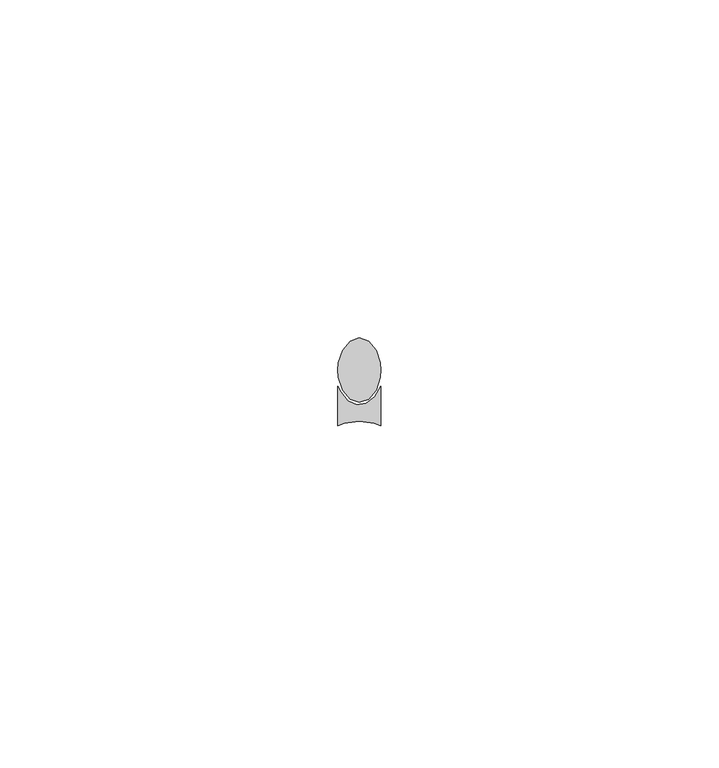
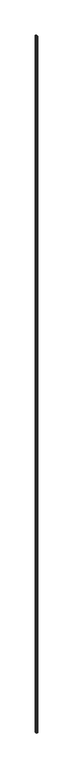
"""IFC4 building model written with IfcOpenShell, lengths in millimetres: proxy geometry, Generic Models 11:Generic Models 1:306267:Generic Models 1:306267 : Generic Models 11:Generic Models 1:306267:300405:Generic Models 1:306267:Generic Models 1:306267 : Generic Models 11:Generic Models 1:306267:300405 : Generic Models 11:Generic Models 1:306267:Generic Models 1:306267 : Generic Models 11:Generic Models 1:306267:300405:4 : Generic Models 11:Generic Models 1:306267:Generic Models 1:306267 : Generic Models 11:Generic Models 1:306267:300405:Generic Models 1:306267:Generic Models 1:306267 : Generic Models 11:Generic Models 1:306267:300405 : Generic Models 11:Generic Models 1:306267:Generic Models 1:306267 : Generic Models 11:Generic Models 1:306267:300405:300182."""

from ifc_helpers import new_model, si_unit, origin, origin_with_axes, place, context, project, spatial, polyline, outline, extrude, source, transform, mapped, element, save


def generic_models_39942859(model_context):
    return source(origin(), model_context, "Body", "SweptSolid", [
        extrude(outline(polyline([(570448.0841431, -579092.0005286), (570446.979409, -579090.6790346), (570446.3663278, -579088.7694203), (570446.2867239, -579087.7096644), (570446.3663278, -579086.6499084), (570446.979409, -579084.7402942), (570448.0841431, -579083.4188002), (570449.4617239, -579082.9471644), (570450.8393048, -579083.4188002), (570451.9440389, -579084.7402942), (570452.5571201, -579086.6499084), (570452.6367239, -579087.7096644), (570452.5571201, -579088.7694203), (570451.9440389, -579090.6790346), (570450.8393048, -579092.0005286), (570449.4617239, -579092.4721644), (570448.0841431, -579092.0005286)])), origin_with_axes(), (0.0, 0.0, 1.0), 3695.7),
        extrude(outline(polyline([(570451.6709607, -579095.5639755), (570449.4617239, -579095.2502894), (570447.2524872, -579095.5639755), (570446.2867239, -579095.9413841), (570446.2867239, -579090.073292), (570446.6730415, -579090.9335729), (570447.756527, -579092.2431481), (570449.1067747, -579092.8435016), (570450.512551, -579092.6407137), (570451.7539351, -579091.6665087), (570452.6367239, -579090.073292), (570452.6367239, -579095.9413841), (570451.6709607, -579095.5639755)])), origin_with_axes(), (0.0, 0.0, 1.0), 3695.7),
    ])


if __name__ == "__main__":
    model = new_model("IFC4")
    model_context = context("Model", 3, world=origin())
    ifc_project = project(units=[si_unit("LENGTHUNIT", "METRE", prefix="MILLI")], contexts=[model_context])
    site = spatial("IfcSite", under=ifc_project)
    building = spatial("IfcBuilding", under=site)
    placement = place(None, origin())
    generic_models_shape = generic_models_39942859(model_context)
    element("IfcBuildingElementProxy", 1, Name="Generic Models 11:Generic Models 1:306267:Generic Models 1:306267 : Generic Models 11:Generic Models 1:306267:300405:Generic Models 1:306267:Generic Models 1:306267 : Generic Models 11:Generic Models 1:306267:300405 : Generic Models 11:Generic Models 1:306267:Generic Models 1:306267 : Generic Models 11:Generic Models 1:306267:300405:4 : Generic Models 11:Generic Models 1:306267:Generic Models 1:306267 : Generic Models 11:Generic Models 1:306267:300405:Generic Models 1:306267:Generic Models 1:306267 : Generic Models 11:Generic Models 1:306267:300405 : Generic Models 11:Generic Models 1:306267:Generic Models 1:306267 : Generic Models 11:Generic Models 1:306267:300405:300182", ObjectType="Generic Models 11:Generic Models 1:306267:Generic Models 1:306267 : Generic Models 11:Generic Models 1:306267:300405:Generic Models 1:306267:Generic Models 1:306267 : Generic Models 11:Generic Models 1:306267:300405 : Generic Models 11:Generic Models 1:306267:Generic Models 1:306267 : Generic Models 11:Generic Models 1:306267:300405:4 : Generic Models 11:Generic Models 1:306267:Generic Models 1:306267 : Generic Models 11:Generic Models 1:306267:300405:Generic Models 1:306267:Generic Models 1:306267 : Generic Models 11:Generic Models 1:306267:300405 : Generic Models 11:Generic Models 1:306267:Generic Models 1:306267 : Generic Models 11:Generic Models 1:306267:300405:300182", at=placement, inside=building, context=model_context, shape_type="MappedRepresentation", body=[
        mapped(generic_models_shape, transform((0.0, 0.0, 0.0), x_axis=(1.0, 0.0, 0.0), y_axis=(0.0, 1.0, 0.0), z_axis=(0.0, 0.0, 1.0))),
    ])
    save(model, "model.ifc")

# Revit data of these elements
# Type "Generic Models 11:Generic Models 1:306267:Generic Models 1:306267 : Generic Models 11:Generic Models 1:306267:300405:Generic Models 1:306267:Generic Models 1:306267 : Generic Models 11:Generic Models 1:306267:300405 : Generic Models 11:Generic Models 1:306267:Generic Models 1:306267 : Generic Models 11:Generic Models 1:306267:300405:4 : Generic Models 11:Generic Models 1:306267:Generic Models 1:306267 : Generic Models 11:Generic Models 1:306267:300405:Generic Models 1:306267:Generic Models 1:306267 : Generic Models 11:Generic Models 1:306267:300405 : Generic Models 11:Generic Models 1:306267:Generic Models 1:306267 : Generic Models 11:Generic Models 1:306267:300405:300182"
#   NameOverride = "Generic Models 11:Generic Models 1:306267:Generic Models 1:306267 : Generic Models 11:Generic Models 1:306267:300405:Generic Models 1:306267:Generic Models 1:306267 : Generic Models 11:Generic Models 1:306267:300405 : Generic Models 11:Generic Models 1:306267:Generic Models 1:306267 : Generic Models 11:Generic Models 1:306267:300405:300182"
#   ObjectTypeOverride = "Generic Models 1:306267:Generic Models 1:306267 : Generic Models 11:Generic Models 1:306267:300405 : Generic Models 11:Generic Models 1:306267:Generic Models 1:306267 : Generic Models 11:Generic Models 1:306267:300405"
#   Reference = "Generic Models 1"
#   Tag = "300182"
# Element 1 (IfcBuildingElementProxy, "Generic Models 11:Generic Models 1:306267:Generic Models 1:306267 : Generic Models 11:Generic Models 1:306267:300405:Generic Models 1:306267:Generic Models 1:306267 : Generic Models 11:Generic Models 1:306267:300405 : Generic Models 11:Generic Models 1:306267:Generic Models 1:306267 : Generic Models 11:Generic Models 1:306267:300405:4 : Generic Models 11:Generic Models 1:306267:Generic Models 1:306267 : Generic Models 11:Generic Models 1:306267:300405:Generic Models 1:306267:Generic Models 1:306267 : Generic Models 11:Generic Models 1:306267:300405 : Generic Models 11:Generic Models 1:306267:Generic Models 1:306267 : Generic Models 11:Generic Models 1:306267:300405:300182")
#   Materials on its faces: "SEALANT & BACKER ROD, IF NECESSARY"
# Materials
#   "SEALANT & BACKER ROD, IF NECESSARY": class "Unassigned", colour RGB 120 120 120, transparency 0, Cost = 0
